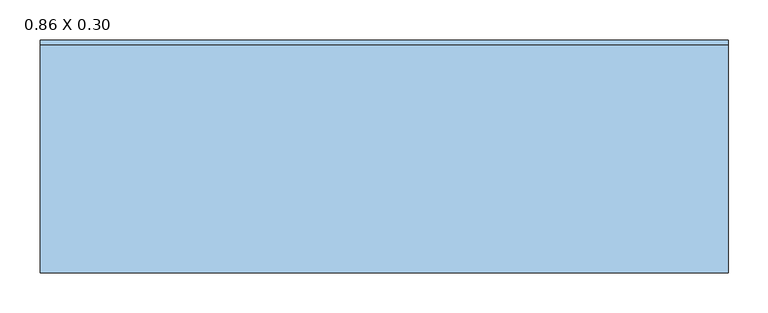
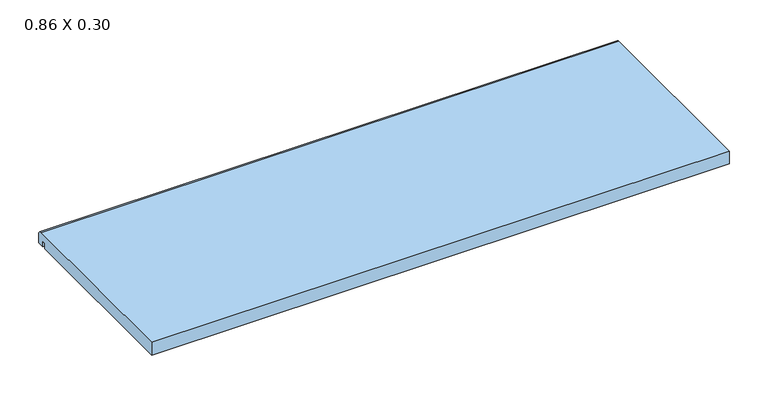
"""IFC4 building model written with IfcOpenShell, lengths in millimetres: window geometry, .CC_ND 300_PEDRA_PEITORIL RETO : 0.86 X 0.30."""

from ifc_helpers import new_model, si_unit, point, frame, frame_2d, origin, place, context, project, spatial, polyline, circle_curve, trimmed, segment, composite_curve, outline, extrude, source, transform, mapped, element, save


def window_0_86_x_0_30_ebf489ac(model_context):
    return source(origin(), model_context, "Body", "SweptSolid", [
        extrude(outline(composite_curve([segment(polyline([(132.5083081, 1480.0), (-143.7, 1480.0), (-143.7, 1500.0), (141.3808343, 1500.0)]), True, "CONTINUOUS"), segment(trimmed(circle_curve(frame_2d((141.3808343, 1493.3808343)), 6.6191657), [point((141.3808343, 1500.0))], [point((148.0, 1493.3808343))], False, "CARTESIAN"), True, "CONTINUOUS"), segment(polyline([(148.0, 1493.3808343), (148.0, 1480.0), (137.2619526, 1480.0), (137.2619526, 1488.1993124), (132.5083081, 1488.1993124), (132.5083081, 1480.0)]), True, "CONTINUOUS")], self_intersect=False)), frame((-430.0, 0.0, 0.0), z_axis=(1.0, 0.0, 0.0), x_axis=(0.0, 1.0, 0.0)), (0.0, 0.0, 1.0), 860.0),
    ])


if __name__ == "__main__":
    model = new_model("IFC4")
    model_context = context("Model", 3, world=origin())
    ifc_project = project(units=[si_unit("LENGTHUNIT", "METRE", prefix="MILLI")], contexts=[model_context])
    site = spatial("IfcSite", under=ifc_project)
    building = spatial("IfcBuilding", under=site)
    placement = place(None, origin())
    window_0_86_x_0_30_shape = window_0_86_x_0_30_ebf489ac(model_context)
    element("IfcWindow", 1, ObjectType=".CC_ND 300_PEDRA_PEITORIL RETO : 0.86 X 0.30", at=placement, inside=building, context=model_context, shape_type="MappedRepresentation", body=[
        mapped(window_0_86_x_0_30_shape, transform((0.0, 0.0, 0.0), x_axis=(1.0, 0.0, 0.0), y_axis=(0.0, 1.0, 0.0), z_axis=(0.0, 0.0, 1.0))),
    ])
    save(model, "model.ifc")

# Revit data of these elements
# Type ".CC_ND 300_PEDRA_PEITORIL RETO : 0.86 X 0.30"
#   Type Mark = "66"
#   Largura da pedra [instance default] = 0.26 m
#   Extensão interior peitoril [instance default] = 0.03 m
#   Extensão exterior peitoril [instance default] = 0.03 m
#   Espessura = 0.02 m
#   Comprimento = 0.86 m
#   Altura-padrão do peitoril = 1.48 m
#   Peitoril = .GRANITO_BRANCO_ITAUNAS
#   Rough Width = 0
#   Rough Height = 0
#   Height = 0
#   Wall Closure = (empty or 0)
#   Width = 0
# Element 1 (IfcWindow, ".CC_ND 300_PEDRA_PEITORIL RETO : 0.86 X 0.30")
#   Largura da pedra = 0.2917 m
#   Extensão interior peitoril = 0.0257 m
#   Materials on its faces: ".GRANITO_BRANCO_ITAUNAS"
# Materials
#   ".GRANITO_BRANCO_ITAUNAS": class ".CC_PEDRA REVEST.", colour RGB 202 195 174, transparency 0, Description = "Revestimento em granito", Cost = 0
